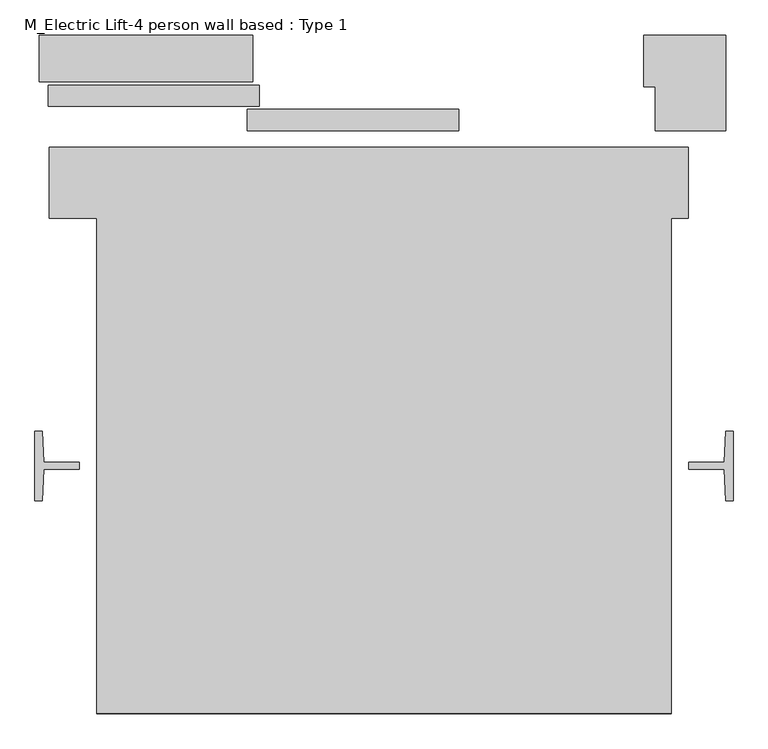
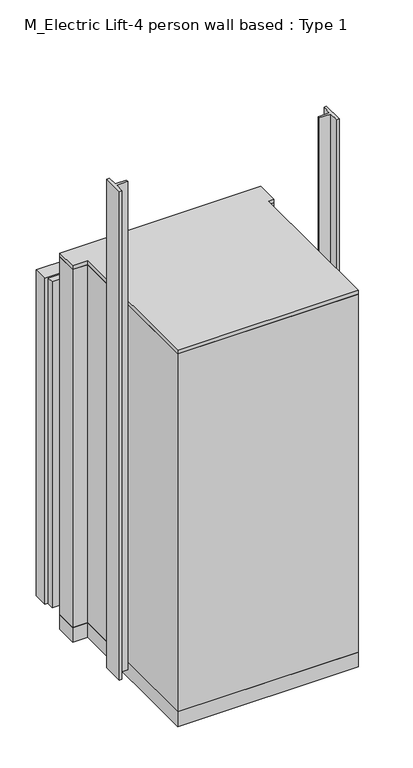
"""IFC4 building model written with IfcOpenShell, lengths in millimetres: proxy geometry, M_Electric Lift-4 person wall based : Type 1."""

import ifcopenshell
import ifcopenshell.guid

model = None  # the IFC model being written
_history = None  # IfcOwnerHistory: only IFC2X3 demands one
_inside = {}  # id of a spatial element -> (the spatial element, [elements in it])
_under = {}  # id of a project, library or spatial element -> (it, [spatial elements below it])
_declared = {}  # id of a project -> (the project, [libraries it declares])
_typed = {}  # id of a type object -> (the type object, [elements of that type])
_made_of = {}  # id of a material, layer set ... -> (it, [elements and type objects made of it])


def new_model(schema):
    """Start an empty IFC model of exactly this schema.

    Asked for "IFC4X3", IfcOpenShell would pick the latest addendum, in which some entities
    have other attributes; the version numbers below select the first issue.
    IFC2X3 requires an IfcOwnerHistory on every rooted entity: one is made here for all.
    """
    global model, _history
    if schema == "IFC4X3":
        model = ifcopenshell.file(schema_version=(4, 3, 0, 0))
    else:
        model = ifcopenshell.file(schema=schema)
    _inside.clear()
    _under.clear()
    _declared.clear()
    _typed.clear()
    _made_of.clear()
    _history = None
    if model.schema == "IFC2X3":
        org = make("IfcOrganization", Name="unknown")
        user = make(
            "IfcPersonAndOrganization",
            ThePerson=make("IfcPerson", FamilyName="unknown"),
            TheOrganization=org,
        )
        app = make(
            "IfcApplication",
            ApplicationDeveloper=org,
            Version="unknown",
            ApplicationFullName="unknown",
            ApplicationIdentifier="unknown",
        )
        _history = make(
            "IfcOwnerHistory",
            OwningUser=user,
            OwningApplication=app,
            ChangeAction="ADDED",
            CreationDate=0,
        )
    return model


def make(cls, **values):
    """One entity of the class cls with the attributes given. An attribute that is None is left unset."""
    return model.create_entity(
        cls, **{name: value for name, value in values.items() if value is not None}
    )


def rooted(cls, **values):
    """An entity with a GlobalId (a new one), such as an element, a storey or a relation."""
    return make(cls, GlobalId=ifcopenshell.guid.new(), OwnerHistory=_history, **values)


def si_unit(unit_type, name, prefix=None):
    """IfcSIUnit, for example si_unit("LENGTHUNIT", "METRE", prefix="MILLI")."""
    return make("IfcSIUnit", UnitType=unit_type, Prefix=prefix, Name=name)


def assignment(units):
    """IfcUnitAssignment: the units of a project."""
    return None if units is None else make("IfcUnitAssignment", Units=units)


def point(xyz):
    """IfcCartesianPoint."""
    return None if xyz is None else make("IfcCartesianPoint", Coordinates=xyz)


def direction(xyz):
    """IfcDirection."""
    return None if xyz is None else make("IfcDirection", DirectionRatios=xyz)


def frame(location, z_axis=None, x_axis=None):
    """IfcAxis2Placement3D, a coordinate frame: its origin and axes. An axis left out is left unset."""
    return make(
        "IfcAxis2Placement3D",
        Location=point(location),
        Axis=direction(z_axis),
        RefDirection=direction(x_axis),
    )


def origin():
    """The frame at (0, 0, 0) with its axes left unset."""
    return frame((0.0, 0.0, 0.0))


def origin_with_axes():
    """The frame at (0, 0, 0) with the z axis (0, 0, 1) and the x axis (1, 0, 0) written out."""
    return frame((0.0, 0.0, 0.0), z_axis=(0.0, 0.0, 1.0), x_axis=(1.0, 0.0, 0.0))


def place(relative_to, where):
    """IfcLocalPlacement: puts the frame where relative to a parent placement (None: the world)."""
    return make(
        "IfcLocalPlacement", PlacementRelTo=relative_to, RelativePlacement=where
    )


def context(
    kind, dimensions, precision=None, world=None, true_north=None, identifier=None
):
    """IfcGeometricRepresentationContext, for example the 3D "Model" context."""
    return make(
        "IfcGeometricRepresentationContext",
        ContextIdentifier=identifier,
        ContextType=kind,
        CoordinateSpaceDimension=dimensions,
        Precision=precision,
        WorldCoordinateSystem=world,
        TrueNorth=true_north,
    )


def project(units=None, contexts=None):
    """IfcProject with its units and contexts."""
    return rooted(
        "IfcProject",
        Name="project",
        RepresentationContexts=contexts,
        UnitsInContext=assignment(units),
    )


def spatial(cls, under=None, at=None, **own):
    """A site, building, storey or space (cls), placed at a placement, below another one or the project."""
    s = rooted(cls, ObjectPlacement=at, **own)
    if under is not None:
        _under.setdefault(under.id(), (under, []))[1].append(s)
    return s


def polyline(points):
    """IfcPolyline through the points."""
    return make("IfcPolyline", Points=[point(p) for p in points])


def outline(outer, holes=None, kind="AREA"):
    """IfcArbitraryClosedProfileDef: a profile drawn as a closed curve; with holes, ...WithVoids."""
    if holes is None:
        return make("IfcArbitraryClosedProfileDef", ProfileType=kind, OuterCurve=outer)
    return make(
        "IfcArbitraryProfileDefWithVoids",
        ProfileType=kind,
        OuterCurve=outer,
        InnerCurves=holes,
    )


def extrude(swept, where, along, depth):
    """IfcExtrudedAreaSolid: the profile swept, set in the frame where, extruded along a direction by depth."""
    return make(
        "IfcExtrudedAreaSolid",
        SweptArea=swept,
        Position=where,
        ExtrudedDirection=direction(along),
        Depth=depth,
    )


def faces_of(points, faces, orient=None, outer=None):
    """IfcFace entities. A face is a list of loops; a loop is a list of indices into points, from 0.

    orient and outer hold one flag for each loop. By default every Orientation is true, the
    first loop of a face is its IfcFaceOuterBound and the others are IfcFaceBound.
    """
    made = []
    for i, loops in enumerate(faces):
        bounds = []
        for j, loop in enumerate(loops):
            is_outer = j == 0 if outer is None else outer[i][j]
            bounds.append(
                make(
                    "IfcFaceOuterBound" if is_outer else "IfcFaceBound",
                    Bound=make("IfcPolyLoop", Polygon=[points[k] for k in loop]),
                    Orientation=True if orient is None else orient[i][j],
                )
            )
        made.append(make("IfcFace", Bounds=bounds))
    return made


def faceted_brep(points, faces, orient=None, outer=None, voids=None):
    """IfcFacetedBrep: a solid bounded by flat faces; with voids (closed shells), ...WithVoids."""
    shared = [point(p) for p in points]
    hull = make("IfcClosedShell", CfsFaces=faces_of(shared, faces, orient, outer))
    if voids is None:
        return make("IfcFacetedBrep", Outer=hull)
    return make(
        "IfcFacetedBrepWithVoids",
        Outer=hull,
        Voids=[
            make(cls, CfsFaces=faces_of(shared, fs, o, b)) for cls, fs, o, b in voids
        ],
    )


def shape(context_of_items, identifier, shape_type, items):
    """IfcShapeRepresentation: the items that make up one representation, for example the "Body"."""
    return make(
        "IfcShapeRepresentation",
        ContextOfItems=context_of_items,
        RepresentationIdentifier=identifier,
        RepresentationType=shape_type,
        Items=items,
    )


def source(mapping_origin, context_of_items, identifier, shape_type, items):
    """IfcRepresentationMap: a shape defined once, which mapped items show again and again."""
    return make(
        "IfcRepresentationMap",
        MappingOrigin=mapping_origin,
        MappedRepresentation=shape(context_of_items, identifier, shape_type, items),
    )


def transform(
    local_origin,
    x_axis=None,
    y_axis=None,
    z_axis=None,
    scale=None,
    scale2=None,
    scale3=None,
    uniform=True,
):
    """IfcCartesianTransformationOperator3D, or its non-uniform kind. x_axis, y_axis, z_axis: its Axis1, 2, 3."""
    if uniform:
        return make(
            "IfcCartesianTransformationOperator3D",
            Axis1=direction(x_axis),
            Axis2=direction(y_axis),
            LocalOrigin=point(local_origin),
            Scale=scale,
            Axis3=direction(z_axis),
        )
    return make(
        "IfcCartesianTransformationOperator3DnonUniform",
        Axis1=direction(x_axis),
        Axis2=direction(y_axis),
        LocalOrigin=point(local_origin),
        Scale=scale,
        Axis3=direction(z_axis),
        Scale2=scale2,
        Scale3=scale3,
    )


def mapped(mapping_source, mapping_target):
    """IfcMappedItem: shows the shape of a source again, moved by a transform."""
    return make(
        "IfcMappedItem", MappingSource=mapping_source, MappingTarget=mapping_target
    )


def made_of(thing, what):
    """Note that an element or type object is made of a material, layer set ...; save() writes the relation."""
    if what is not None:
        _made_of.setdefault(what.id(), (what, []))[1].append(thing)
    return thing


def element(
    cls,
    number,
    at=None,
    inside=None,
    cuts=None,
    type_object=None,
    material=None,
    context=None,
    identifier="Body",
    shape_type=None,
    held_by="IfcProductDefinitionShape",
    body=None,
    shapes=None,
    **own,
):
    """One element of the class cls, such as IfcWall. Its Tag is "e" and its number.

    at: its placement. inside: the storey or other place that contains it. cuts: it is an
    opening in that element (IfcRelVoidsElement). A single representation is given by context,
    identifier, shape_type and body (its items); several are given by shapes. held_by: the class
    of the entity that holds the representations. save() writes the other relations.
    """
    e = rooted(cls, Tag="e%d" % number, ObjectPlacement=at, **own)
    if body is not None:
        shapes = [shape(context, identifier, shape_type, body)]
    if shapes is not None:
        e.Representation = make(held_by, Representations=shapes)
    if inside is not None:
        _inside.setdefault(inside.id(), (inside, []))[1].append(e)
    if cuts is not None:
        rooted(
            "IfcRelVoidsElement", RelatingBuildingElement=cuts, RelatedOpeningElement=e
        )
    if type_object is not None:
        _typed.setdefault(type_object.id(), (type_object, []))[1].append(e)
    return made_of(e, material)


def aggregate(whole, parts):
    """IfcRelAggregates: a whole, such as a stair, and the parts it consists of."""
    return rooted("IfcRelAggregates", RelatingObject=whole, RelatedObjects=parts)


def save(model, path):
    """Write the relations noted so far, then the file.

    IfcRelAggregates (storeys below a building ...), IfcRelContainedInSpatialStructure (elements
    in a storey), IfcRelDefinesByType, IfcRelAssociatesMaterial and IfcRelDeclares: one each for
    every whole, place, type object, material and project.
    """
    for whole, parts in _under.values():
        aggregate(whole, parts)
    for where, things in _inside.values():
        rooted(
            "IfcRelContainedInSpatialStructure",
            RelatedElements=things,
            RelatingStructure=where,
        )
    for kind, things in _typed.values():
        rooted("IfcRelDefinesByType", RelatedObjects=things, RelatingType=kind)
    for what, things in _made_of.values():
        rooted("IfcRelAssociatesMaterial", RelatedObjects=things, RelatingMaterial=what)
    for by, libraries in _declared.values():
        rooted("IfcRelDeclares", RelatingContext=by, RelatedDefinitions=libraries)
    model.write(path)


def m_electric_lift_4_person_wall_based_type_1_25105fba(model_context):
    return source(origin(), model_context, "Body", "SolidModel", [
        extrude(outline(polyline([(-400.0, -1140.0000001), (-400.0, -235.0), (-486.5, -235.0), (-486.5, -105.0), (681.0, -105.0), (681.0, -235.0), (650.0, -235.0), (650.0, -1140.0000001), (-400.0, -1140.0000001)])), frame((0.0, 0.0, 2200.0), z_axis=(0.0, 0.0, 1.0), x_axis=(1.0, 0.0, 0.0)), (0.0, 0.0, 1.0), 22.0),
        extrude(outline(polyline([(-448.6220553, -190.9893804), (-448.6220553, -149.3893804), (-62.6220553, -149.3893804), (-62.6220553, -190.9893804), (-448.6220553, -190.9893804)])), origin_with_axes(), (0.0, 0.0, 1.0), 2000.0),
        extrude(outline(polyline([(-114.8301, -144.0), (-114.8301, -108.9587126), (271.1699, -108.9587126), (271.1699, -144.0), (-114.8301, -144.0)])), origin_with_axes(), (0.0, 0.0, 1.0), 2000.0),
        extrude(outline(polyline([(-488.6220553, 8.3893803), (-102.6220553, 8.3893803), (-102.6220553, -30.6106197), (-488.6220553, -30.6106197), (-488.6220553, 8.3893803)])), origin_with_axes(), (0.0, 0.0, 1.0), 2000.0),
        extrude(outline(polyline([(-124.8301, -75.0), (-124.8301, -36.0), (261.1699, -36.0), (261.1699, -75.0), (-124.8301, -75.0)])), origin_with_axes(), (0.0, 0.0, 1.0), 2000.0),
        extrude(outline(polyline([(-400.0, -1140.0000001), (-400.0, -235.0), (-486.5, -235.0), (-486.5, -105.0), (681.0, -105.0), (681.0, -235.0), (650.0, -235.0), (650.0, -1140.0000001), (-400.0, -1140.0000001)])), frame((0.0, 0.0, -90.0), z_axis=(0.0, 0.0, 1.0), x_axis=(1.0, 0.0, 0.0)), (0.0, 0.0, 1.0), 90.0),
        faceted_brep([(-400.0, -1140.0000001, 2200.0), (650.0, -1140.0000001, 2200.0), (650.0, -235.0, 2200.0), (681.0, -235.0, 2200.0), (681.0, -105.0, 2200.0), (-486.5, -105.0, 2200.0), (-486.5, -235.0, 2200.0), (-400.0, -235.0, 2200.0), (-375.0, -1115.0000001, 2200.0), (-375.0, -235.0, 2200.0), (-110.3, -235.0, 2200.0), (-110.3, -197.0, 2200.0), (-458.1228936, -197.0, 2200.0), (-458.1228936, -108.9587126, 2200.0), (621.1699, -108.9587126, 2200.0), (621.1699, -192.6835257, 2200.0), (600.0, -192.6835257, 2200.0), (600.0, -235.0, 2200.0), (625.0, -235.0, 2200.0), (625.0, -572.5016433, 2200.0), (610.2454439, -572.5016433, 2200.0), (610.2454439, -802.5016433, 2200.0), (625.0, -802.5016433, 2200.0), (625.0, -1115.0000001, 2200.0), (-400.0, -1140.0000001, 0.0), (-400.0, -235.0, 0.0), (-486.5, -235.0, 0.0), (-486.5, -105.0, 0.0), (-173.4437103, -105.0, 0.0), (-173.4437103, -108.9587126, 0.0), (-458.1228936, -108.9587126, 0.0), (-458.1228936, -197.0, 0.0), (-110.3, -197.0, 0.0), (-110.3, -235.0, 0.0), (-375.0, -235.0, 0.0), (-375.0, -1115.0000001, 0.0), (625.0, -1115.0000001, 0.0), (625.0, -802.5016433, 0.0), (610.2454439, -802.5016433, 0.0), (610.2454439, -572.5016433, 0.0), (625.0, -572.5016433, 0.0), (625.0, -235.0, 0.0), (600.0, -235.0, 0.0), (600.0, -192.6835257, 0.0), (621.1699, -192.6835257, 0.0), (621.1699, -105.0, 0.0), (681.0, -105.0, 0.0), (681.0, -235.0, 0.0), (650.0, -235.0, 0.0), (650.0, -1140.0000001, 0.0), (621.1699, -105.0, 2000.0), (-173.4437103, -105.0, 2000.0), (-173.4437103, -108.9587126, 2000.0), (621.1699, -108.9587126, 2000.0), (600.0, -192.6835257, 2000.0)], [[[0, 1, 2, 3, 4, 5, 6, 7], [8, 9, 10, 11, 12, 13, 14, 15, 16, 17, 18, 19, 20, 21, 22, 23]], [[24, 25, 26, 27, 28, 29, 30, 31, 32, 33, 34, 35, 36, 37, 38, 39, 40, 41, 42, 43, 44, 45, 46, 47, 48, 49]], [[1, 0, 24, 49]], [[2, 1, 49, 48]], [[3, 2, 48, 47]], [[4, 3, 47, 46]], [[5, 4, 46, 45, 50, 51, 28, 27]], [[6, 5, 27, 26]], [[7, 6, 26, 25]], [[0, 7, 25, 24]], [[9, 8, 35, 34]], [[10, 9, 34, 33]], [[11, 10, 33, 32]], [[12, 11, 32, 31]], [[13, 12, 31, 30]], [[14, 13, 30, 29, 52, 53]], [[15, 14, 53, 50, 45, 44]], [[16, 15, 44, 43, 54]], [[17, 16, 54, 43, 42]], [[18, 17, 42, 41]], [[19, 18, 41, 40]], [[20, 19, 40, 39]], [[21, 20, 39, 38]], [[22, 21, 38, 37]], [[23, 22, 37, 36]], [[8, 23, 36, 35]], [[50, 53, 52, 51]], [[51, 52, 29, 28]]]),
        extrude(outline(polyline([(750.026988, -751.0012199), (747.026988, -693.80122), (682.0269884, -693.80122), (682.0269884, -681.3056039), (747.1132057, -681.3056039), (750.026988, -624.0012199), (763.026988, -624.0012199), (763.026988, -751.0012199), (750.026988, -751.0012199)])), origin_with_axes(), (0.0, 0.0, 1.0), 3000.0),
        extrude(outline(polyline([(-497.026988, -693.80122), (-500.026988, -751.0012199), (-513.026988, -751.0012199), (-513.026988, -624.0012199), (-500.026988, -624.0012199), (-497.1132057, -681.3056039), (-432.0269884, -681.3056039), (-432.0269884, -693.80122), (-497.026988, -693.80122)])), origin_with_axes(), (0.0, 0.0, 1.0), 3000.0),
        extrude(outline(polyline([(-114.9791786, 100.0), (-114.9791786, 14.4785696), (-505.0067971, 14.4785696), (-505.0067971, 100.0), (-114.9791786, 100.0)])), origin_with_axes(), (0.0, 0.0, 1.0), 2000.0),
        extrude(outline(polyline([(600.0, 5.0), (600.0, 100.0), (750.0, 100.0), (750.0, -75.0), (621.1699, -75.0), (621.1699, 5.0), (600.0, 5.0)])), origin_with_axes(), (0.0, 0.0, 1.0), 2000.0),
    ])


if __name__ == "__main__":
    model = new_model("IFC4")
    model_context = context("Model", 3, world=origin())
    ifc_project = project(units=[si_unit("LENGTHUNIT", "METRE", prefix="MILLI")], contexts=[model_context])
    site = spatial("IfcSite", under=ifc_project)
    building = spatial("IfcBuilding", under=site)
    placement = place(None, origin())
    m_electric_lift_4_person_wall_based_type_1_shape = m_electric_lift_4_person_wall_based_type_1_25105fba(model_context)
    element("IfcBuildingElementProxy", 1, Name="M_Electric Lift-4 person wall based : Type 1", ObjectType="M_Electric Lift-4 person wall based : Type 1", at=placement, inside=building, context=model_context, shape_type="MappedRepresentation", body=[
        mapped(m_electric_lift_4_person_wall_based_type_1_shape, transform((0.0, 0.0, 0.0), x_axis=(1.0, 0.0, 0.0), y_axis=(0.0, 1.0, 0.0), z_axis=(0.0, 0.0, 1.0))),
    ])
    save(model, "model.ifc")

# Revit data of these elements
# Type "M_Electric Lift-4 person wall based : Type 1"
#   Door Material = none
#   Manufacturer = ""
#   Default Elevation = 0
#   Assembly Code = ""
